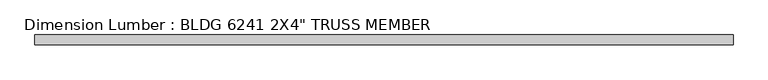
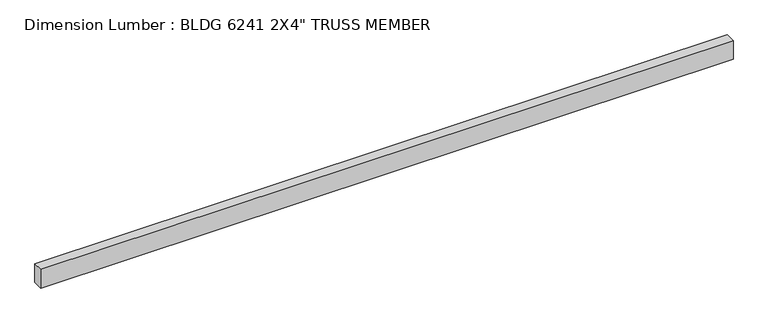
"""IFC4 building model written with IfcOpenShell, lengths in millimetres: beam geometry."""

from ifc_helpers import new_model, si_unit, frame, origin, place, context, project, spatial, polyline, outline, extrude, source, transform, mapped, element, save


def beam_5a6f5897(model_context):
    return source(origin(), model_context, "Body", "SweptSolid", [
        extrude(outline(polyline([(1795.057951, 25.4), (1795.057951, -25.4), (-1769.657951, -25.4), (-1769.657951, 25.4), (1795.057951, 25.4)])), frame((0.0, 0.0, -50.8), z_axis=(0.0, 0.0, 1.0), x_axis=(1.0, 0.0, 0.0)), (0.0, 0.0, 1.0), 101.6),
    ])


if __name__ == "__main__":
    model = new_model("IFC4")
    model_context = context("Model", 3, world=origin())
    ifc_project = project(units=[si_unit("LENGTHUNIT", "METRE", prefix="MILLI")], contexts=[model_context])
    site = spatial("IfcSite", under=ifc_project)
    building = spatial("IfcBuilding", under=site)
    placement = place(None, origin())
    beam_shape = beam_5a6f5897(model_context)
    element("IfcBeam", 1, ObjectType="Dimension Lumber : BLDG 6241 2X4\" TRUSS MEMBER", at=placement, inside=building, context=model_context, shape_type="MappedRepresentation", body=[
        mapped(beam_shape, transform((0.0, 0.0, 0.0), x_axis=(1.0, 0.0, 0.0), y_axis=(0.0, 1.0, 0.0), z_axis=(0.0, 0.0, 1.0))),
    ])
    save(model, "model.ifc")

# Revit data of these elements
# Type "Dimension Lumber : BLDG 6241 2X4\" TRUSS MEMBER"
#   Assembly Code = "B10"
#   A = 0.273472 SF
#   Length [instance default] = 5' - 0"
#   b = 0' - 2"
#   d = 0' - 4"
#   Structural Material [instance default] = Softwood, Lumber
# Element 1 (IfcBeam, "Dimension Lumber : BLDG 6241 2X4\" TRUSS MEMBER")
#   Materials on its faces: "Softwood, Lumber"
# Materials
#   "Softwood, Lumber": class "Wood", colour RGB 223 192 134, transparency 0, Description = "Pinus Echinata", Cost = 0
